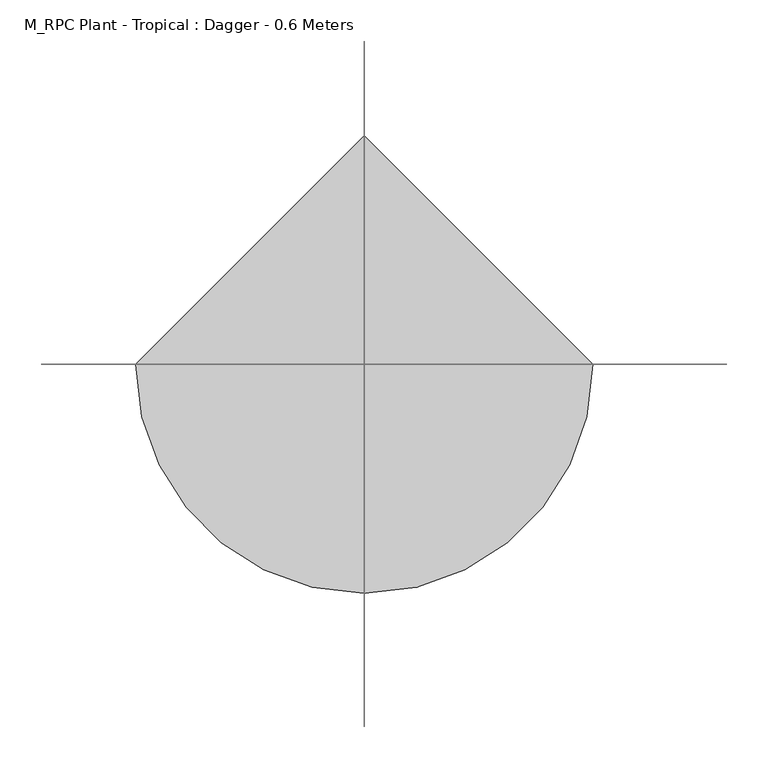
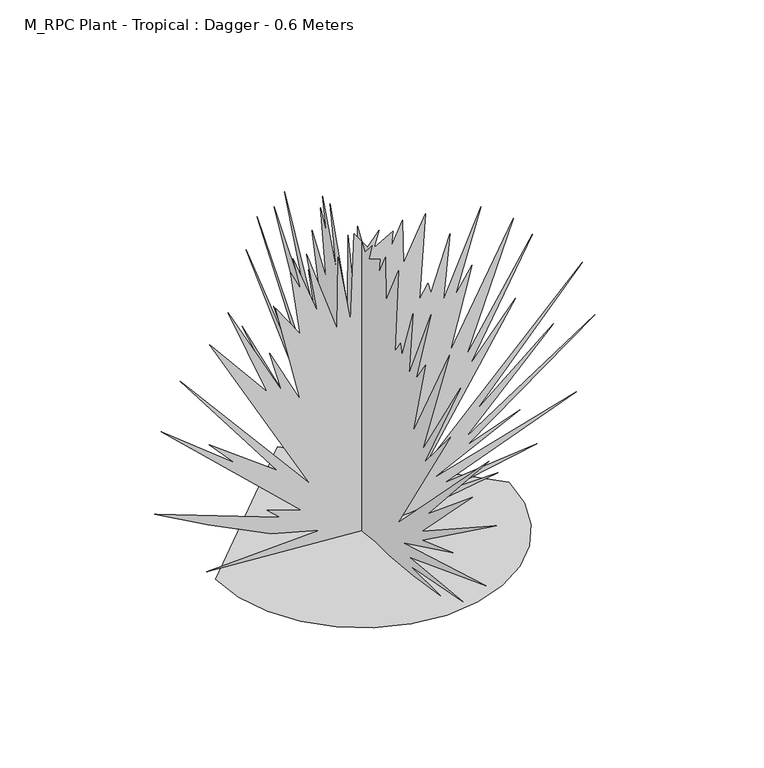
"""IFC4 building model written with IfcOpenShell, lengths in millimetres: geographic element geometry, M_RPC Plant - Tropical : Dagger - 0.6 Meters."""

from ifc_helpers import new_model, si_unit, origin, place, context, project, spatial, triangles, source, transform, mapped, element, save


def m_rpc_plant_tropical_dagger_0_6_meters_3415abb8(model_context):
    return source(origin(), model_context, "Body", "Tessellation", [
        triangles([(0.1799897, -5.7252047, 0.0), (0.1800089, 294.2752427, 20.8333418), (0.1799966, 80.3860635, 29.1667744), (0.1800035, 172.052634, 54.1667927), (0.1800144, 292.8852294, 115.2778473), (0.1800237, 392.885321, 170.8333952), (0.1800042, 155.3861186, 81.9445621), (0.180007, 180.386137, 104.166834), (0.1800018, 115.1083446, 81.9445621), (0.1800325, 380.3853209, 331.9452544), (0.1800176, 241.4971961, 220.8334319), (0.1800237, 290.1077282, 273.610225), (0.1800103, 160.9416298, 177.7779023), (0.1800356, 344.2752794, 419.4453278), (0.1800038, 99.8305798, 130.555603), (0.1800355, 288.7202402, 473.6103719), (0.1800212, 180.386137, 341.6677714), (0.1800365, 253.9977048, 525.00044), (0.1800191, 152.6083812, 334.7227738), (0.1800253, 174.8306439, 416.6678447), (0.1800152, 117.8860911, 304.167753), (0.1800298, 163.7193854, 502.7779229), (0.1800231, 117.8860911, 436.1103353), (0.1800318, 135.9416114, 563.8904717), (0.1800283, 116.4970952, 525.00044), (0.180033, 130.3861093, 590.2779599), (0.180023, 84.5525697, 468.0553694), (0.1800315, 105.3860819, 590.2779599), (0.1800179, 47.0527875, 420.8328521), (0.1800264, 45.663787, 563.8904717), (0.1800169, 22.052617, 427.7778497), (0.1800267, 15.1081371, 600.0004769), (0.1800231, -9.8918086, 563.8904717), (0.1800233, -32.1140259, 590.2779599), (0.180022, -22.3918427, 558.3329621), (0.1800211, -58.503047, 579.1679549), (0.1800196, -55.7252959, 551.3904353), (0.1800209, -76.5585628, 594.4454744), (0.1800157, -77.9475587, 508.3329254), (0.1800183, -119.6140924, 593.0554793), (0.1800089, -108.5030882, 425.0003303), (0.1800095, -125.1698489, 451.3903619), (0.180008, -130.7253601, 430.5553328), (0.1800121, -166.8363826, 536.110445), (0.1800052, -154.3363825, 408.3328156), (0.1800106, -225.1696861, 569.4454742), (0.180004, -176.5586453, 411.1103351), (0.180005, -208.5031707, 458.3328524), (0.179998, -166.8363826, 300.0002385), (0.1800043, -286.2802365, 525.00044), (0.1799951, -197.3919122, 281.9452359), (0.1799995, -322.3927488, 480.5554058), (0.1799934, -204.3364192, 261.1102067), (0.1799944, -290.4477329, 363.8902885), (0.1799882, -118.2253418, 87.5000733), (0.1799886, -416.8378198, 391.6678082), (0.1799871, -215.4476778, 165.277884), (0.1799856, -362.6703049, 287.5002384), (0.1799854, -196.0031525, 118.0555938), (0.1799804, -440.4478612, 277.7777214), (0.1799843, -198.7809081, 101.3890784), (0.1799804, -298.7802366, 137.5001101), (0.1799855, -134.8918572, 58.333299), (0.179974, -405.725344, 136.1111142), (0.1799833, -155.7253784, 41.6667836), (0.1799738, -330.7252707, 58.333299), (0.1799822, -157.11412, 25.0000206), (0.1799763, -257.1152108, 26.3890211), (0.1799808, -168.2253785, 12.5000103), (0.1799851, -87.669567, 4.1666533), (0.1799877, -43.2252867, 4.1666533), (-277.616067, 0.0, 0.0922626), (-270.2710575, -63.6563025, 0.0922626), (-249.3550376, -122.1146029, 0.0922626), (-216.5405072, -173.699899, 0.0922626), (-173.5032359, -216.7371703, 0.0922626), (-121.9179307, -249.5517008, 0.0922626), (-63.4596303, -270.4677206, 0.0922626), (0.1966832, -277.8127301, 0.0922626), (63.8529748, -270.4677206, 0.0922626), (122.3112752, -249.5517008, 0.0922626), (173.8965621, -216.7371703, 0.0922626), (216.9338335, -173.699899, 0.0922626), (249.7483639, -122.1146029, 0.0922626), (270.6643837, -63.6563025, 0.0922626), (278.0093933, 2.43e-05, 0.0922626), (0.1966346, 277.8127301, 0.0922626), (5.9218758, 0.016681, 0.0), (-294.0785796, 0.0166798, 20.8333418), (-80.1893913, 0.0166793, 29.1667744), (-171.8562252, 0.0166778, 54.1667927), (-292.6885663, 0.0166741, 115.2778473), (-392.6886397, 0.0166708, 170.8333952), (-155.1894555, 0.0166761, 81.9445621), (-180.1894738, 0.0166748, 104.166834), (-114.9116723, 0.0166761, 81.9445621), (-380.1886396, 0.0166612, 331.9452544), (-241.3005329, 0.0166679, 220.8334319), (-289.9110651, 0.0166647, 273.610225), (-160.7449667, 0.0166704, 177.7779023), (-344.0785981, 0.016656, 419.4453278), (-99.6339076, 0.0166732, 130.555603), (-288.5235771, 0.0166528, 473.6103719), (-180.1894738, 0.0166607, 341.6677714), (-253.8010417, 0.0166497, 525.00044), (-152.411718, 0.0166611, 334.7227738), (-174.6339808, 0.0166562, 416.6678447), (-117.6894188, 0.0166629, 304.167753), (-163.5227222, 0.016651, 502.7779229), (-117.6894188, 0.016655, 436.1103353), (-135.7449392, 0.0166474, 563.8904717), (-116.300423, 0.0166497, 525.00044), (-130.1894371, 0.0166458, 590.2779599), (-84.3558975, 0.0166531, 468.0553694), (-105.1894097, 0.0166458, 590.2779599), (-46.8561152, 0.0166559, 420.8328521), (-45.4671148, 0.0166474, 563.8904717), (-21.855947, 0.0166555, 427.7778497), (-14.911491, 0.0166453, 600.0004769), (10.0885046, 0.0166474, 563.8904717), (32.3106959, 0.0166458, 590.2779599), (22.5885127, 0.0166477, 558.3329621), (58.6997192, 0.0166465, 579.1679549), (55.9219681, 0.0166481, 551.3904353), (76.755235, 0.0166456, 594.4454744), (78.1442309, 0.0166507, 508.3329254), (119.8107646, 0.0166457, 593.0554793), (108.6997604, 0.0166557, 425.0003303), (125.3665211, 0.0166541, 451.3903619), (130.9220323, 0.0166553, 430.5553328), (167.0330458, 0.0166491, 536.110445), (154.5330457, 0.0166567, 408.3328156), (225.3663493, 0.0166471, 569.4454742), (176.7553084, 0.0166565, 411.1103351), (208.6998339, 0.0166537, 458.3328524), (167.0330458, 0.0166631, 300.0002385), (286.4768997, 0.0166497, 525.00044), (197.5885753, 0.0166642, 281.9452359), (322.5894301, 0.0166524, 480.5554058), (204.5330824, 0.0166655, 261.1102067), (290.644396, 0.0166593, 363.8902885), (118.422014, 0.0166758, 87.5000733), (417.0345011, 0.0166577, 391.6678082), (215.6443409, 0.0166712, 165.277884), (362.8669862, 0.0166639, 287.5002384), (196.1998156, 0.016674, 118.0555938), (440.6445425, 0.0166645, 277.7777214), (198.9775712, 0.016675, 101.3890784), (298.9768998, 0.0166728, 137.5001101), (135.0885294, 0.0166776, 58.333299), (405.9220253, 0.0166729, 136.1111142), (155.9220416, 0.0166785, 41.6667836), (330.9219521, 0.0166776, 58.333299), (157.3107831, 0.0166795, 25.0000206), (257.3118739, 0.0166795, 26.3890211), (168.4220417, 0.0166803, 12.5000103), (87.8662392, 0.0166808, 4.1666533), (43.4219589, 0.0166808, 4.1666533)], [[68, 67, 69], [69, 67, 70], [64, 63, 65], [62, 61, 63], [58, 57, 59], [56, 55, 57], [57, 55, 59], [52, 51, 53], [50, 49, 51], [48, 47, 49], [46, 45, 47], [47, 45, 49], [40, 39, 41], [36, 35, 37], [34, 33, 35], [28, 27, 29], [26, 25, 27], [24, 23, 25], [22, 21, 23], [20, 19, 21], [16, 15, 17], [12, 11, 13], [10, 9, 11], [11, 9, 13], [8, 7, 9], [2, 1, 3], [66, 65, 67], [67, 65, 70], [65, 63, 70], [60, 59, 61], [61, 59, 63], [59, 55, 63], [63, 55, 70], [54, 53, 55], [53, 51, 55], [51, 49, 55], [49, 45, 55], [44, 43, 45], [45, 43, 55], [43, 42, 55], [42, 41, 55], [55, 41, 70], [41, 39, 70], [70, 39, 71], [39, 38, 71], [38, 37, 71], [37, 35, 71], [71, 35, 1], [35, 33, 1], [33, 32, 1], [18, 17, 19], [17, 15, 19], [19, 15, 21], [14, 13, 15], [13, 9, 15], [6, 5, 7], [5, 4, 7], [4, 3, 7], [7, 3, 9], [9, 3, 15], [21, 15, 23], [23, 15, 25], [25, 15, 27], [15, 3, 27], [27, 3, 29], [3, 1, 29], [29, 1, 30], [30, 1, 31], [1, 32, 31], [86, 87, 72], [85, 86, 72], [85, 72, 73], [84, 85, 73], [84, 73, 74], [84, 74, 75], [83, 84, 75], [82, 83, 75], [82, 75, 76], [82, 76, 77], [82, 77, 78], [82, 78, 79], [82, 79, 80], [82, 80, 81], [154, 155, 156], [154, 156, 157], [150, 151, 152], [148, 149, 150], [144, 145, 146], [142, 143, 144], [142, 144, 146], [138, 139, 140], [136, 137, 138], [134, 135, 136], [132, 133, 134], [132, 134, 136], [126, 127, 128], [122, 123, 124], [120, 121, 122], [114, 115, 116], [112, 113, 114], [110, 111, 112], [108, 109, 110], [106, 107, 108], [102, 103, 104], [98, 99, 100], [96, 97, 98], [96, 98, 100], [94, 95, 96], [88, 89, 90], [152, 153, 154], [152, 154, 157], [150, 152, 157], [146, 147, 148], [146, 148, 150], [142, 146, 150], [142, 150, 157], [140, 141, 142], [138, 140, 142], [136, 138, 142], [132, 136, 142], [130, 131, 132], [130, 132, 142], [129, 130, 142], [128, 129, 142], [128, 142, 157], [126, 128, 157], [126, 157, 158], [125, 126, 158], [124, 125, 158], [122, 124, 158], [122, 158, 88], [120, 122, 88], [119, 120, 88], [104, 105, 106], [102, 104, 106], [102, 106, 108], [100, 101, 102], [96, 100, 102], [92, 93, 94], [91, 92, 94], [90, 91, 94], [90, 94, 96], [90, 96, 102], [102, 108, 110], [102, 110, 112], [102, 112, 114], [90, 102, 114], [90, 114, 116], [88, 90, 116], [88, 116, 117], [88, 117, 118], [119, 88, 118]], closed=False),
    ])


if __name__ == "__main__":
    model = new_model("IFC4")
    model_context = context("Model", 3, world=origin())
    ifc_project = project(units=[si_unit("LENGTHUNIT", "METRE", prefix="MILLI")], contexts=[model_context])
    site = spatial("IfcSite", under=ifc_project)
    building = spatial("IfcBuilding", under=site)
    placement = place(None, origin())
    m_rpc_plant_tropical_dagger_0_6_meters_shape = m_rpc_plant_tropical_dagger_0_6_meters_3415abb8(model_context)
    element("IfcGeographicElement", 1, ObjectType="M_RPC Plant - Tropical : Dagger - 0.6 Meters", at=placement, inside=building, context=model_context, shape_type="MappedRepresentation", body=[
        mapped(m_rpc_plant_tropical_dagger_0_6_meters_shape, transform((0.0, 0.0, 0.0), x_axis=(1.0, 0.0, 0.0), y_axis=(0.0, 1.0, 0.0), z_axis=(0.0, 0.0, 1.0))),
    ])
    save(model, "model.ifc")

# Revit data of these elements
# Type "M_RPC Plant - Tropical : Dagger - 0.6 Meters"
#   built-in parameter 1005198 = "{2, 15},{39, RPC-16-G3A7-NEG0-UH6H-J000-ST1L-LVER-AU},{1, 0},{1, 0},{2, 35},{1, 8},{5, Color},{1, 0},{1, 0},{3, 0.8},{3, 0.8},{3, 0.8},{1, 8},{7, BBoxMin},{1, 0},{1, 0},{1, 0},{1, 0},{1, 0},{1, 8},{7, BBoxMax},{1, 0},{1, 0},{1, 0},{1, 0},{1, 0},{2, 11},{9, RPCTypeId},{1, 0},{1, 0},{39, RPC-16-G3A7-NEG0-UH6H-J000-ST1L-LVER-AU},{1, 6},{14, RPCPlantHeight},{1, 0},{1, 0},{6, 1.9685},{2, 11},{7, keyword},{1, 0},{1, 0},{55, :Geometry:RPC:Dagger:Yucca Recurvifolia:plant:tropical.},{2, 11},{8, category},{1, 0},{1, 0},{17, :Plants [General]},{2, 11},{12, LocalizedUID},{1, 0},{1, 0},{6, Dagger},{2, 14},{6, Height},{1, 0},{1, 0},{6, 1.9685},{1, 2},{16, Cast Reflections},{1, 0},{1, 0},{1, 0},{1, 2},{12, Cast Shadows},{1, 0},{1, 0},{1, 1},{1, 2},{9, Lock View},{1, 0},{1, 0},{1, 0},{1, 4},{5, ViewC},{1, 0},{1, 0},{1, 0},{2, 11},{20, AdvancedUIDefinition},{1, 0},{1, 0},{0, },{2, 11},{10, AssetLibID},{1, 0},{1, 0},{36, 4D3F6E72-3F99-4203-98E9-AF80B3C7A7A4},{2, 11},{10, BaseSchema},{1, 0},{1, 0},{9, RPCSchema},{2, 11},{12, ExchangeGUID},{1, 0},{1, 0},{0, },{1, 2},{6, Hidden},{1, 0},{1, 0},{1, 0},{1, 4},{11, RPCCategory},{1, 0},{1, 0},{1, 0},{2, 11},{8, RPCImage},{1, 0},{1, 0},{0, },{1, 4},{13, SchemaVersion},{1, 0},{1, 0},{1, 4},{2, 11},{12, UIDefinition},{1, 0},{1, 0},{0, },{2, 11},{6, UIName},{1, 0},{1, 0},{39, RPC-16-G3A7-NEG0-UH6H-J000-ST1L-LVER-AU},{2, 11},{11, VersionGUID},{1, 0},{1, 0},{9, RPCSchema},{2, 11},{9, assettype},{1, 0},{1, 0},{11, RPCGeometry},{2, 11},{11, description},{1, 0},{1, 0},{0, },{2, 11},{9, localname},{1, 0},{1, 0},{3, RPC},{2, 11},{9, localtype},{1, 0},{1, 0},{3, RPC},{1, 4},{8, revision},{1, 0},{1, 0},{1, 1},{2, 11},{9, thumbnail},{1, 0},{1, 0},{0, },{1, 4},{7, version},{1, 0},{1, 0},{1, 1},{1, 2},{20, RPC_Cast Reflections},{1, 0},{1, 0},{1, 1},{1, 2},{16, RPC_Cast Shadows},{1, 0},{1, 0},{1, 1},{1, 2},{13, RPC_Lock View},{1, 0},{1, 0},{1, 0},{1, 4},{9, RPC_ViewC},{1, 0},{1, 0},{1, 0},{21, assetlibrary_base.fbx},{1, 5},"
#   built-in parameter 1005195 = "RPC-16-G3A7-NEG0-UH6H-J000-ST1L-LVER-AU"
#   Type Comments = "Dagger"
#   Height = 0.6 m
#   Description = (empty or 0)
#   Default Elevation = 0
